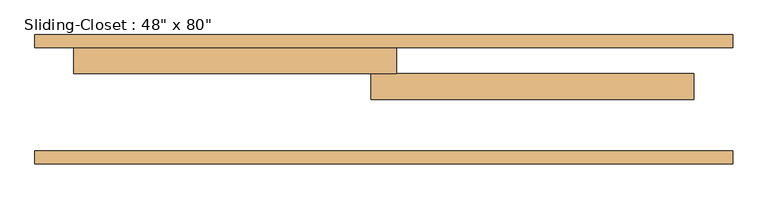
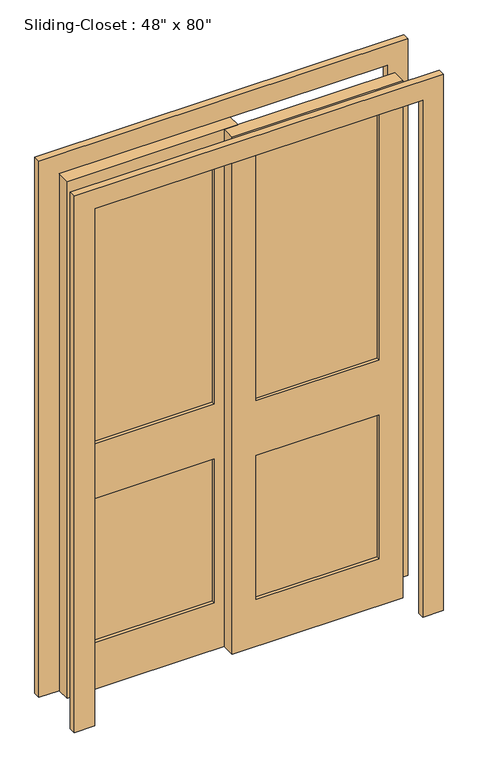
"""IFC4 building model written with IfcOpenShell, lengths in millimetres: door geometry."""

from ifc_helpers import new_model, si_unit, frame, origin, place, context, project, spatial, polyline, outline, extrude, source, transform, mapped, element, save


def door_5d877b8f(model_context):
    return source(origin(), model_context, "Body", "SweptSolid", [
        extrude(outline(polyline([(-63.5, 190.5), (-520.7, 190.5), (-520.7, 215.9), (-63.5, 215.9), (-63.5, 190.5)])), frame((0.0, 0.0, 965.2), z_axis=(0.0, 0.0, 1.0), x_axis=(1.0, 0.0, 0.0)), (0.0, 0.0, 1.0), 977.9),
        extrude(outline(polyline([(-63.5, 190.5), (-520.7, 190.5), (-520.7, 215.9), (-63.5, 215.9), (-63.5, 190.5)])), frame((0.0, 0.0, 184.15), z_axis=(0.0, 0.0, 1.0), x_axis=(1.0, 0.0, 0.0)), (0.0, 0.0, 1.0), 565.15),
        extrude(outline(polyline([(63.5, 165.1), (520.7, 165.1), (520.7, 139.7), (63.5, 139.7), (63.5, 165.1)])), frame((0.0, 0.0, 965.2), z_axis=(0.0, 0.0, 1.0), x_axis=(1.0, 0.0, 0.0)), (0.0, 0.0, 1.0), 977.9),
        extrude(outline(polyline([(63.5, 165.1), (520.7, 165.1), (520.7, 139.7), (63.5, 139.7), (63.5, 165.1)])), frame((0.0, 0.0, 184.15), z_axis=(0.0, 0.0, 1.0), x_axis=(1.0, 0.0, 0.0)), (0.0, 0.0, 1.0), 565.15),
        extrude(outline(polyline([(2032.0, 25.4), (2032.0, -609.6), (0.0, -609.6), (0.0, 25.4), (2032.0, 25.4)]), holes=[polyline([(184.15, -520.7), (749.3, -520.7), (749.3, -63.5), (184.15, -63.5), (184.15, -520.7)]), polyline([(965.2, -520.7), (1943.1, -520.7), (1943.1, -63.5), (965.2, -63.5), (965.2, -520.7)])]), frame((0.0, 177.8, 0.0), z_axis=(0.0, 1.0, 0.0), x_axis=(0.0, 0.0, 1.0)), (0.0, 0.0, 1.0), 50.8),
        extrude(outline(polyline([(0.0, -685.8), (0.0, -609.6), (2032.0, -609.6), (2032.0, 609.6), (0.0, 609.6), (0.0, 685.8), (2108.2, 685.8), (2108.2, -685.8), (0.0, -685.8)])), frame((0.0, 0.0, 0.0), z_axis=(0.0, 1.0, 0.0), x_axis=(0.0, 0.0, 1.0)), (0.0, 0.0, 1.0), 25.4),
        extrude(outline(polyline([(0.0, 685.8), (2108.2, 685.8), (2108.2, -685.8), (0.0, -685.8), (0.0, -609.6), (2032.0, -609.6), (2032.0, 609.6), (0.0, 609.6), (0.0, 685.8)])), frame((0.0, 228.6, 0.0), z_axis=(0.0, 1.0, 0.0), x_axis=(0.0, 0.0, 1.0)), (0.0, 0.0, 1.0), 25.4),
        extrude(outline(polyline([(2032.0, -25.4), (0.0, -25.4), (0.0, 609.6), (2032.0, 609.6), (2032.0, -25.4)]), holes=[polyline([(965.2, 520.7), (965.2, 63.5), (1943.1, 63.5), (1943.1, 520.7), (965.2, 520.7)]), polyline([(184.15, 520.7), (184.15, 63.5), (749.3, 63.5), (749.3, 520.7), (184.15, 520.7)])]), frame((0.0, 127.0, 0.0), z_axis=(0.0, 1.0, 0.0), x_axis=(0.0, 0.0, 1.0)), (0.0, 0.0, 1.0), 50.8),
    ])


if __name__ == "__main__":
    model = new_model("IFC4")
    model_context = context("Model", 3, world=origin())
    ifc_project = project(units=[si_unit("LENGTHUNIT", "METRE", prefix="MILLI")], contexts=[model_context])
    site = spatial("IfcSite", under=ifc_project)
    building = spatial("IfcBuilding", under=site)
    placement = place(None, origin())
    door_shape = door_5d877b8f(model_context)
    element("IfcDoor", 1, ObjectType="Sliding-Closet : 48\" x 80\"", at=placement, inside=building, context=model_context, shape_type="MappedRepresentation", body=[
        mapped(door_shape, transform((0.0, 0.0, 0.0), x_axis=(1.0, 0.0, 0.0), y_axis=(0.0, 1.0, 0.0), z_axis=(0.0, 0.0, 1.0))),
    ])
    save(model, "model.ifc")

# Revit data of these elements
# Type "Sliding-Closet : 48\" x 80\""
#   Type Mark = "54"
#   Assembly Code = "C1020"
#   Thickness = 0' - 2"
#   Height = 6' - 8"
#   Trim Projection Ext = 0' - 1"
#   Trim Projection Int = 0' - 1"
#   Trim Width = 0' - 3"
#   Width = 4' - 0"
#   Define Thermal Properties by = 0
#   Function = 0
#   Door Material = Door - Panel
#   Frame Material = Door - Frame
#   Wall Closure = (empty or 0)
# Element 1 (IfcDoor, "Sliding-Closet : 48\" x 80\"")
#   Materials on its faces: "Door - Panel", "Door - Frame"
# Materials
#   "Door - Panel": class "Wood", colour RGB 227 170 128, transparency 0, Cost = 0
#   "Door - Frame": class "Miscellaneous", colour RGB 153 76 43, transparency 0, Cost = 0
